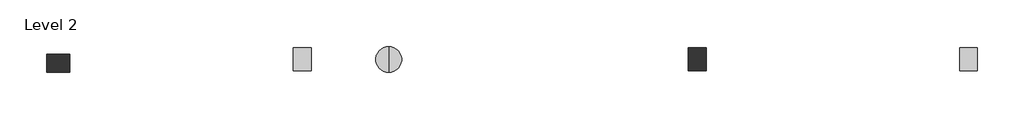
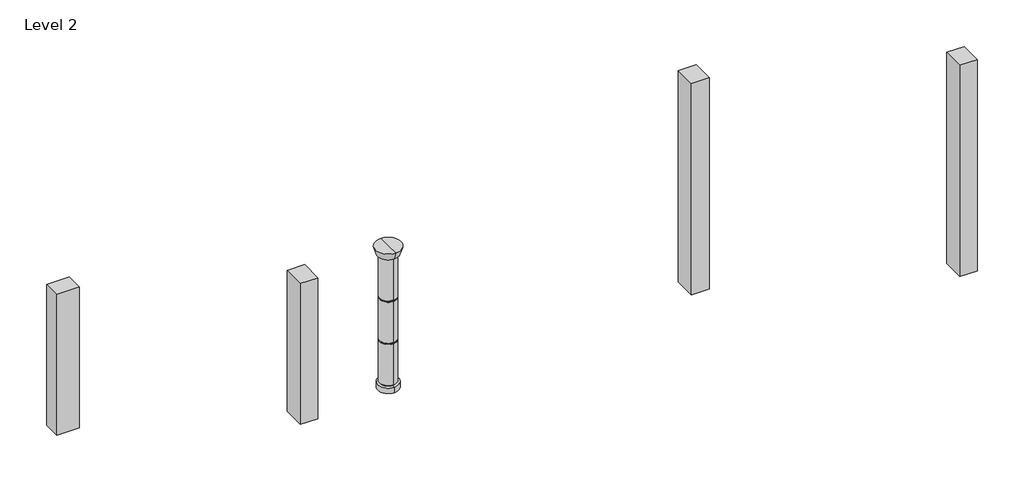
# One storey: 5 columns.
"""IFC4 building model written with IfcOpenShell, lengths in millimetres."""

import ifcopenshell
import ifcopenshell.guid

model = None  # the IFC model being written
_history = None  # IfcOwnerHistory: only IFC2X3 demands one
_inside = {}  # id of a spatial element -> (the spatial element, [elements in it])
_under = {}  # id of a project, library or spatial element -> (it, [spatial elements below it])
_declared = {}  # id of a project -> (the project, [libraries it declares])
_typed = {}  # id of a type object -> (the type object, [elements of that type])
_made_of = {}  # id of a material, layer set ... -> (it, [elements and type objects made of it])


def new_model(schema):
    """Start an empty IFC model of exactly this schema.

    Asked for "IFC4X3", IfcOpenShell would pick the latest addendum, in which some entities
    have other attributes; the version numbers below select the first issue.
    IFC2X3 requires an IfcOwnerHistory on every rooted entity: one is made here for all.
    """
    global model, _history
    if schema == "IFC4X3":
        model = ifcopenshell.file(schema_version=(4, 3, 0, 0))
    else:
        model = ifcopenshell.file(schema=schema)
    _inside.clear()
    _under.clear()
    _declared.clear()
    _typed.clear()
    _made_of.clear()
    _history = None
    if model.schema == "IFC2X3":
        org = make("IfcOrganization", Name="unknown")
        user = make(
            "IfcPersonAndOrganization",
            ThePerson=make("IfcPerson", FamilyName="unknown"),
            TheOrganization=org,
        )
        app = make(
            "IfcApplication",
            ApplicationDeveloper=org,
            Version="unknown",
            ApplicationFullName="unknown",
            ApplicationIdentifier="unknown",
        )
        _history = make(
            "IfcOwnerHistory",
            OwningUser=user,
            OwningApplication=app,
            ChangeAction="ADDED",
            CreationDate=0,
        )
    return model


def make(cls, **values):
    """One entity of the class cls with the attributes given. An attribute that is None is left unset."""
    return model.create_entity(
        cls, **{name: value for name, value in values.items() if value is not None}
    )


def rooted(cls, **values):
    """An entity with a GlobalId (a new one), such as an element, a storey or a relation."""
    return make(cls, GlobalId=ifcopenshell.guid.new(), OwnerHistory=_history, **values)


def si_unit(unit_type, name, prefix=None):
    """IfcSIUnit, for example si_unit("LENGTHUNIT", "METRE", prefix="MILLI")."""
    return make("IfcSIUnit", UnitType=unit_type, Prefix=prefix, Name=name)


def assignment(units):
    """IfcUnitAssignment: the units of a project."""
    return None if units is None else make("IfcUnitAssignment", Units=units)


def point(xyz):
    """IfcCartesianPoint."""
    return None if xyz is None else make("IfcCartesianPoint", Coordinates=xyz)


def direction(xyz):
    """IfcDirection."""
    return None if xyz is None else make("IfcDirection", DirectionRatios=xyz)


def frame(location, z_axis=None, x_axis=None):
    """IfcAxis2Placement3D, a coordinate frame: its origin and axes. An axis left out is left unset."""
    return make(
        "IfcAxis2Placement3D",
        Location=point(location),
        Axis=direction(z_axis),
        RefDirection=direction(x_axis),
    )


def origin():
    """The frame at (0, 0, 0) with its axes left unset."""
    return frame((0.0, 0.0, 0.0))


def origin_with_axes():
    """The frame at (0, 0, 0) with the z axis (0, 0, 1) and the x axis (1, 0, 0) written out."""
    return frame((0.0, 0.0, 0.0), z_axis=(0.0, 0.0, 1.0), x_axis=(1.0, 0.0, 0.0))


def place(relative_to, where):
    """IfcLocalPlacement: puts the frame where relative to a parent placement (None: the world)."""
    return make(
        "IfcLocalPlacement", PlacementRelTo=relative_to, RelativePlacement=where
    )


def context(
    kind, dimensions, precision=None, world=None, true_north=None, identifier=None
):
    """IfcGeometricRepresentationContext, for example the 3D "Model" context."""
    return make(
        "IfcGeometricRepresentationContext",
        ContextIdentifier=identifier,
        ContextType=kind,
        CoordinateSpaceDimension=dimensions,
        Precision=precision,
        WorldCoordinateSystem=world,
        TrueNorth=true_north,
    )


def project(units=None, contexts=None):
    """IfcProject with its units and contexts."""
    return rooted(
        "IfcProject",
        Name="project",
        RepresentationContexts=contexts,
        UnitsInContext=assignment(units),
    )


def spatial(cls, under=None, at=None, **own):
    """A site, building, storey or space (cls), placed at a placement, below another one or the project."""
    s = rooted(cls, ObjectPlacement=at, **own)
    if under is not None:
        _under.setdefault(under.id(), (under, []))[1].append(s)
    return s


def polyline(points):
    """IfcPolyline through the points."""
    return make("IfcPolyline", Points=[point(p) for p in points])


def circle_curve(where, radius):
    """IfcCircle in the frame where."""
    return make("IfcCircle", Position=where, Radius=radius)


def outline(outer, holes=None, kind="AREA"):
    """IfcArbitraryClosedProfileDef: a profile drawn as a closed curve; with holes, ...WithVoids."""
    if holes is None:
        return make("IfcArbitraryClosedProfileDef", ProfileType=kind, OuterCurve=outer)
    return make(
        "IfcArbitraryProfileDefWithVoids",
        ProfileType=kind,
        OuterCurve=outer,
        InnerCurves=holes,
    )


def extrude(swept, where, along, depth):
    """IfcExtrudedAreaSolid: the profile swept, set in the frame where, extruded along a direction by depth."""
    return make(
        "IfcExtrudedAreaSolid",
        SweptArea=swept,
        Position=where,
        ExtrudedDirection=direction(along),
        Depth=depth,
    )


def shape(context_of_items, identifier, shape_type, items):
    """IfcShapeRepresentation: the items that make up one representation, for example the "Body"."""
    return make(
        "IfcShapeRepresentation",
        ContextOfItems=context_of_items,
        RepresentationIdentifier=identifier,
        RepresentationType=shape_type,
        Items=items,
    )


def source(mapping_origin, context_of_items, identifier, shape_type, items):
    """IfcRepresentationMap: a shape defined once, which mapped items show again and again."""
    return make(
        "IfcRepresentationMap",
        MappingOrigin=mapping_origin,
        MappedRepresentation=shape(context_of_items, identifier, shape_type, items),
    )


def transform(
    local_origin,
    x_axis=None,
    y_axis=None,
    z_axis=None,
    scale=None,
    scale2=None,
    scale3=None,
    uniform=True,
):
    """IfcCartesianTransformationOperator3D, or its non-uniform kind. x_axis, y_axis, z_axis: its Axis1, 2, 3."""
    if uniform:
        return make(
            "IfcCartesianTransformationOperator3D",
            Axis1=direction(x_axis),
            Axis2=direction(y_axis),
            LocalOrigin=point(local_origin),
            Scale=scale,
            Axis3=direction(z_axis),
        )
    return make(
        "IfcCartesianTransformationOperator3DnonUniform",
        Axis1=direction(x_axis),
        Axis2=direction(y_axis),
        LocalOrigin=point(local_origin),
        Scale=scale,
        Axis3=direction(z_axis),
        Scale2=scale2,
        Scale3=scale3,
    )


def mapped(mapping_source, mapping_target):
    """IfcMappedItem: shows the shape of a source again, moved by a transform."""
    return make(
        "IfcMappedItem", MappingSource=mapping_source, MappingTarget=mapping_target
    )


def made_of(thing, what):
    """Note that an element or type object is made of a material, layer set ...; save() writes the relation."""
    if what is not None:
        _made_of.setdefault(what.id(), (what, []))[1].append(thing)
    return thing


def element(
    cls,
    number,
    at=None,
    inside=None,
    cuts=None,
    type_object=None,
    material=None,
    context=None,
    identifier="Body",
    shape_type=None,
    held_by="IfcProductDefinitionShape",
    body=None,
    shapes=None,
    **own,
):
    """One element of the class cls, such as IfcWall. Its Tag is "e" and its number.

    at: its placement. inside: the storey or other place that contains it. cuts: it is an
    opening in that element (IfcRelVoidsElement). A single representation is given by context,
    identifier, shape_type and body (its items); several are given by shapes. held_by: the class
    of the entity that holds the representations. save() writes the other relations.
    """
    e = rooted(cls, Tag="e%d" % number, ObjectPlacement=at, **own)
    if body is not None:
        shapes = [shape(context, identifier, shape_type, body)]
    if shapes is not None:
        e.Representation = make(held_by, Representations=shapes)
    if inside is not None:
        _inside.setdefault(inside.id(), (inside, []))[1].append(e)
    if cuts is not None:
        rooted(
            "IfcRelVoidsElement", RelatingBuildingElement=cuts, RelatedOpeningElement=e
        )
    if type_object is not None:
        _typed.setdefault(type_object.id(), (type_object, []))[1].append(e)
    return made_of(e, material)


def aggregate(whole, parts):
    """IfcRelAggregates: a whole, such as a stair, and the parts it consists of."""
    return rooted("IfcRelAggregates", RelatingObject=whole, RelatedObjects=parts)


def save(model, path):
    """Write the relations noted so far, then the file.

    IfcRelAggregates (storeys below a building ...), IfcRelContainedInSpatialStructure (elements
    in a storey), IfcRelDefinesByType, IfcRelAssociatesMaterial and IfcRelDeclares: one each for
    every whole, place, type object, material and project.
    """
    for whole, parts in _under.values():
        aggregate(whole, parts)
    for where, things in _inside.values():
        rooted(
            "IfcRelContainedInSpatialStructure",
            RelatedElements=things,
            RelatingStructure=where,
        )
    for kind, things in _typed.values():
        rooted("IfcRelDefinesByType", RelatedObjects=things, RelatingType=kind)
    for what, things in _made_of.values():
        rooted("IfcRelAssociatesMaterial", RelatedObjects=things, RelatingMaterial=what)
    for by, libraries in _declared.values():
        rooted("IfcRelDeclares", RelatingContext=by, RelatedDefinitions=libraries)
    model.write(path)


def plane_surface(at):
    """IfcPlane: the flat surface through the origin of the frame at, square to its z axis."""
    return make("IfcPlane", Position=at)


def cylinder_surface(at, radius):
    """IfcCylindricalSurface: all points at the distance radius from the z axis of the frame at."""
    return make("IfcCylindricalSurface", Position=at, Radius=radius)


def revolved_surface(curve, axis_point, axis_direction):
    """IfcSurfaceOfRevolution: the curve turned about the line through axis_point along axis_direction."""
    return make(
        "IfcSurfaceOfRevolution",
        SweptCurve=make("IfcArbitraryOpenProfileDef", ProfileType="CURVE", Curve=curve),
        AxisPosition=make("IfcAxis1Placement", Location=point(axis_point), Axis=direction(axis_direction)),
    )


def advanced_brep(points, edges, surfaces, faces):
    """IfcAdvancedBrep: a solid bounded by faces that lie on surfaces and meet in shared edges.

    An edge is (start, end): straight between two places in points (the first is 0);
    or (start, end, curve); or (start, end, curve, False) where it runs against its curve.
    A face is (place in surfaces, loops), or (place, loops, False) where it looks against
    its surface's normal. A loop lists edges by number (the first is 1), with a minus sign
    where the edge is run from its end to its start. The first loop is the outer one.
    """
    corners = [point(p) for p in points]
    vertices = [make("IfcVertexPoint", VertexGeometry=c) for c in corners]
    made = []
    for start, end, *more in edges:
        made.append(
            make(
                "IfcEdgeCurve",
                EdgeStart=vertices[start],
                EdgeEnd=vertices[end],
                EdgeGeometry=more[0] if more else make("IfcPolyline", Points=[corners[start], corners[end]]),
                SameSense=more[1] if len(more) > 1 else True,
            )
        )
    hull = []
    for where, loops, *sense in faces:
        bounds = []
        for j, loop in enumerate(loops):
            ring = [make("IfcOrientedEdge", EdgeElement=made[abs(k) - 1], Orientation=k > 0) for k in loop]
            bounds.append(
                make(
                    "IfcFaceOuterBound" if j == 0 else "IfcFaceBound",
                    Bound=make("IfcEdgeLoop", EdgeList=ring),
                    Orientation=True,
                )
            )
        hull.append(make("IfcAdvancedFace", Bounds=bounds, FaceSurface=surfaces[where], SameSense=sense[0] if sense else True))
    return make("IfcAdvancedBrep", Outer=make("IfcClosedShell", CfsFaces=hull))


def m_rectangular_column_475_x_610mm_712a9979(model_context):
    return source(origin(), model_context, "Body", "SweptSolid", [
        extrude(outline(polyline([(305.0, 237.5), (305.0, -237.5), (-305.0, -237.5), (-305.0, 237.5), (305.0, 237.5)])), origin_with_axes(), (0.0, 0.0, 1.0), 6000.0),
    ])


def m_rectangular_column_475_x_610mm_a7c237de(model_context):
    return source(origin(), model_context, "Body", "SweptSolid", [
        extrude(outline(polyline([(305.0, 237.5), (305.0, -237.5), (-305.0, -237.5), (-305.0, 237.5), (305.0, 237.5)])), frame((0.0, 0.0, -2000.0), z_axis=(0.0, 0.0, 1.0), x_axis=(1.0, 0.0, 0.0)), (0.0, 0.0, 1.0), 6000.0),
    ])


def m_rectangular_column_475_x_610mm_e62a7db6(model_context):
    return source(origin(), model_context, "Body", "SweptSolid", [
        extrude(outline(polyline([(305.0, 237.5), (305.0, -237.5), (-305.0, -237.5), (-305.0, 237.5), (305.0, 237.5)])), frame((0.0, 0.0, 2000.0), z_axis=(0.0, 0.0, 1.0), x_axis=(1.0, 0.0, 0.0)), (0.0, 0.0, 1.0), 4000.0),
    ])


def m_rectangular_column_475_x_610mm_b7c60445(model_context):
    return source(origin(), model_context, "Body", "SweptSolid", [
        extrude(outline(polyline([(305.0, 237.5), (305.0, -237.5), (-305.0, -237.5), (-305.0, 237.5), (305.0, 237.5)])), origin_with_axes(), (0.0, 0.0, 1.0), 4000.0),
    ])


def column_c029851a(model_context):
    return source(origin(), model_context, "Body", "AdvancedBrep", [
        advanced_brep(
        [(0.0, 0.0, 0.0), (-279.4, 0.0, 0.0), (279.4, 0.0, 0.0), (-279.4, 0.0, 152.4), (279.4, 0.0, 152.4), (203.2, 0.0, 1392.6), (-203.2, 0.0, 1392.6), (-228.6, 0.0, 1392.6), (228.6, 0.0, 1392.6), (-228.6, 0.0, 2556.6), (228.6, 0.0, 2556.6), (203.2, 0.0, 1354.5), (-203.2, 0.0, 1354.5), (228.6, 0.0, 1354.5), (-228.6, 0.0, 1354.5), (228.6, 0.0, 190.5), (-228.6, 0.0, 190.5), (203.2, 0.0, 190.5), (-203.2, 0.0, 190.5), (203.2, 0.0, 152.4), (-203.2, 0.0, 152.4), (279.4, 0.0, 3796.8), (-279.4, 0.0, 3796.8), (-342.9, 0.0, 4000.0), (342.9, 0.0, 4000.0), (0.0, 0.0, 4000.0), (203.2, 0.0, 3796.8), (-203.2, 0.0, 3796.8), (203.2, 0.0, 3758.7), (-203.2, 0.0, 3758.7), (228.6, 0.0, 3758.7), (-228.6, 0.0, 3758.7), (228.6, 0.0, 2594.7), (-228.6, 0.0, 2594.7), (203.2, 0.0, 2594.7), (-203.2, 0.0, 2594.7), (203.2, 0.0, 2556.6), (-203.2, 0.0, 2556.6)],
        [
            (0, 1),
            (1, 2, circle_curve(frame((0.0, 0.0, 0.0), z_axis=(0.0, 0.0, -1.0), x_axis=(-1.0, 0.0, 0.0)), 279.4)),
            (2, 0),
            (2, 1, circle_curve(frame((0.0, 0.0, 0.0), z_axis=(0.0, 0.0, -1.0), x_axis=(-1.0, 0.0, 0.0)), 279.4)),
            (1, 3),
            (3, 4, circle_curve(frame((0.0, 0.0, 152.4), z_axis=(0.0, 0.0, -1.0), x_axis=(-1.0, 0.0, 0.0)), 279.4)),
            (4, 2),
            (4, 3, circle_curve(frame((0.0, 0.0, 152.4), z_axis=(0.0, 0.0, -1.0), x_axis=(-1.0, 0.0, 0.0)), 279.4)),
            (5, 6, circle_curve(frame((0.0, 0.0, 1392.6), z_axis=(0.0, 0.0, 1.0), x_axis=(-1.0, 0.0, 0.0)), 203.2)),
            (6, 7),
            (7, 8, circle_curve(frame((0.0, 0.0, 1392.6), z_axis=(0.0, 0.0, -1.0), x_axis=(-1.0, 0.0, 0.0)), 228.6)),
            (8, 5),
            (7, 9),
            (9, 10, circle_curve(frame((0.0, 0.0, 2556.6), z_axis=(0.0, 0.0, -1.0), x_axis=(-1.0, 0.0, 0.0)), 228.6)),
            (10, 8),
            (7, 8, circle_curve(frame((0.0, 0.0, 1392.6), z_axis=(0.0, 0.0, 1.0), x_axis=(-1.0, 0.0, 0.0)), 228.6)),
            (10, 9, circle_curve(frame((0.0, 0.0, 2556.6), z_axis=(0.0, 0.0, -1.0), x_axis=(-1.0, 0.0, 0.0)), 228.6)),
            (6, 5, circle_curve(frame((0.0, 0.0, 1392.6), z_axis=(0.0, 0.0, 1.0), x_axis=(-1.0, 0.0, 0.0)), 203.2)),
            (11, 12, circle_curve(frame((0.0, 0.0, 1354.5), z_axis=(0.0, 0.0, 1.0), x_axis=(-1.0, 0.0, 0.0)), 203.2)),
            (12, 6),
            (5, 11),
            (12, 11, circle_curve(frame((0.0, 0.0, 1354.5), z_axis=(0.0, 0.0, 1.0), x_axis=(-1.0, 0.0, 0.0)), 203.2)),
            (13, 14, circle_curve(frame((0.0, 0.0, 1354.5), z_axis=(0.0, 0.0, 1.0), x_axis=(-1.0, 0.0, 0.0)), 228.6)),
            (14, 12),
            (11, 13),
            (14, 13, circle_curve(frame((0.0, 0.0, 1354.5), z_axis=(0.0, 0.0, 1.0), x_axis=(-1.0, 0.0, 0.0)), 228.6)),
            (15, 16, circle_curve(frame((0.0, 0.0, 190.5), z_axis=(0.0, 0.0, 1.0), x_axis=(-1.0, 0.0, 0.0)), 228.6)),
            (16, 14),
            (13, 15),
            (16, 15, circle_curve(frame((0.0, 0.0, 190.5), z_axis=(0.0, 0.0, 1.0), x_axis=(-1.0, 0.0, 0.0)), 228.6)),
            (17, 18, circle_curve(frame((0.0, 0.0, 190.5), z_axis=(0.0, 0.0, 1.0), x_axis=(-1.0, 0.0, 0.0)), 203.2)),
            (18, 16),
            (15, 17),
            (18, 17, circle_curve(frame((0.0, 0.0, 190.5), z_axis=(0.0, 0.0, 1.0), x_axis=(-1.0, 0.0, 0.0)), 203.2)),
            (19, 20, circle_curve(frame((0.0, 0.0, 152.4), z_axis=(0.0, 0.0, 1.0), x_axis=(-1.0, 0.0, 0.0)), 203.2)),
            (20, 18),
            (17, 19),
            (20, 19, circle_curve(frame((0.0, 0.0, 152.4), z_axis=(0.0, 0.0, 1.0), x_axis=(-1.0, 0.0, 0.0)), 203.2)),
            (3, 20),
            (19, 4),
            (21, 22, circle_curve(frame((0.0, 0.0, 3796.8), z_axis=(0.0, 0.0, 1.0), x_axis=(-1.0, 0.0, 0.0)), 279.4)),
            (22, 23),
            (23, 24, circle_curve(frame((0.0, 0.0, 4000.0), z_axis=(0.0, 0.0, -1.0), x_axis=(-1.0, 0.0, 0.0)), 342.9)),
            (24, 21),
            (23, 25),
            (25, 24),
            (23, 24, circle_curve(frame((0.0, 0.0, 4000.0), z_axis=(0.0, 0.0, 1.0), x_axis=(-1.0, 0.0, 0.0)), 342.9)),
            (22, 21, circle_curve(frame((0.0, 0.0, 3796.8), z_axis=(0.0, 0.0, 1.0), x_axis=(-1.0, 0.0, 0.0)), 279.4)),
            (26, 27, circle_curve(frame((0.0, 0.0, 3796.8), z_axis=(0.0, 0.0, 1.0), x_axis=(-1.0, 0.0, 0.0)), 203.2)),
            (27, 22),
            (21, 26),
            (27, 26, circle_curve(frame((0.0, 0.0, 3796.8), z_axis=(0.0, 0.0, 1.0), x_axis=(-1.0, 0.0, 0.0)), 203.2)),
            (28, 29, circle_curve(frame((0.0, 0.0, 3758.7), z_axis=(0.0, 0.0, 1.0), x_axis=(-1.0, 0.0, 0.0)), 203.2)),
            (29, 27),
            (26, 28),
            (29, 28, circle_curve(frame((0.0, 0.0, 3758.7), z_axis=(0.0, 0.0, 1.0), x_axis=(-1.0, 0.0, 0.0)), 203.2)),
            (30, 31, circle_curve(frame((0.0, 0.0, 3758.7), z_axis=(0.0, 0.0, 1.0), x_axis=(-1.0, 0.0, 0.0)), 228.6)),
            (31, 29),
            (28, 30),
            (31, 30, circle_curve(frame((0.0, 0.0, 3758.7), z_axis=(0.0, 0.0, 1.0), x_axis=(-1.0, 0.0, 0.0)), 228.6)),
            (32, 33, circle_curve(frame((0.0, 0.0, 2594.7), z_axis=(0.0, 0.0, 1.0), x_axis=(-1.0, 0.0, 0.0)), 228.6)),
            (33, 31),
            (30, 32),
            (33, 32, circle_curve(frame((0.0, 0.0, 2594.7), z_axis=(0.0, 0.0, 1.0), x_axis=(-1.0, 0.0, 0.0)), 228.6)),
            (34, 35, circle_curve(frame((0.0, 0.0, 2594.7), z_axis=(0.0, 0.0, 1.0), x_axis=(-1.0, 0.0, 0.0)), 203.2)),
            (35, 33),
            (32, 34),
            (35, 34, circle_curve(frame((0.0, 0.0, 2594.7), z_axis=(0.0, 0.0, 1.0), x_axis=(-1.0, 0.0, 0.0)), 203.2)),
            (36, 37, circle_curve(frame((0.0, 0.0, 2556.6), z_axis=(0.0, 0.0, 1.0), x_axis=(-1.0, 0.0, 0.0)), 203.2)),
            (37, 35),
            (34, 36),
            (37, 36, circle_curve(frame((0.0, 0.0, 2556.6), z_axis=(0.0, 0.0, 1.0), x_axis=(-1.0, 0.0, 0.0)), 203.2)),
            (9, 37),
            (36, 10),
        ],
        [
            plane_surface(frame((0.0, 0.0, 0.0), z_axis=(0.0, 0.0, -1.0), x_axis=(-1.0, 0.0, 0.0))),
            cylinder_surface(frame((0.0, 0.0, 4000.0), z_axis=(0.0, 0.0, -1.0), x_axis=(-1.0, 0.0, 0.0)), 279.4),
            plane_surface(frame((0.0, 0.0, 1392.6), z_axis=(0.0, 0.0, -1.0), x_axis=(-1.0, 0.0, 0.0))),
            cylinder_surface(frame((0.0, 0.0, 4000.0), z_axis=(0.0, 0.0, -1.0), x_axis=(-1.0, 0.0, 0.0)), 228.6),
            cylinder_surface(frame((0.0, 0.0, 4000.0), z_axis=(0.0, 0.0, -1.0), x_axis=(-1.0, 0.0, 0.0)), 203.2),
            plane_surface(frame((0.0, 0.0, 1354.5), z_axis=(0.0, 0.0, 1.0), x_axis=(-1.0, 0.0, 0.0))),
            plane_surface(frame((0.0, 0.0, 190.5), z_axis=(0.0, 0.0, -1.0), x_axis=(-1.0, 0.0, 0.0))),
            plane_surface(frame((0.0, 0.0, 152.4), z_axis=(0.0, 0.0, 1.0), x_axis=(-1.0, 0.0, 0.0))),
            revolved_surface(polyline([(-342.9, 0.0, 4000.0), (-279.4, 0.0, 3796.8)]), (0.0, 0.0, 4000.0), (0.0, 0.0, -1.0)),
            plane_surface(frame((0.0, 0.0, 4000.0), z_axis=(0.0, 0.0, 1.0), x_axis=(-1.0, 0.0, 0.0))),
            plane_surface(frame((0.0, 0.0, 3796.8), z_axis=(0.0, 0.0, -1.0), x_axis=(-1.0, 0.0, 0.0))),
            plane_surface(frame((0.0, 0.0, 3758.7), z_axis=(0.0, 0.0, 1.0), x_axis=(-1.0, 0.0, 0.0))),
            plane_surface(frame((0.0, 0.0, 2594.7), z_axis=(0.0, 0.0, -1.0), x_axis=(-1.0, 0.0, 0.0))),
            plane_surface(frame((0.0, 0.0, 2556.6), z_axis=(0.0, 0.0, 1.0), x_axis=(-1.0, 0.0, 0.0))),
        ],
        [
            (0, [[1, 2, 3]]),
            (0, [[-3, 4, -1]]),
            (1, [[-2, 5, 6, 7]]),
            (1, [[-4, -7, 8, -5]]),
            (2, [[9, 10, 11, 12]]),
            (3, [[-11, 13, 14, 15]]),
            (3, [[16, -15, 17, -13]]),
            (2, [[18, -12, -16, -10]]),
            (4, [[19, 20, -9, 21]]),
            (4, [[22, -21, -18, -20]]),
            (5, [[23, 24, -19, 25]]),
            (5, [[26, -25, -22, -24]]),
            (3, [[27, 28, -23, 29]]),
            (3, [[30, -29, -26, -28]]),
            (6, [[31, 32, -27, 33]]),
            (6, [[34, -33, -30, -32]]),
            (4, [[35, 36, -31, 37]]),
            (4, [[38, -37, -34, -36]]),
            (7, [[-6, 39, -35, 40]]),
            (7, [[-8, -40, -38, -39]]),
            (8, [[41, 42, 43, 44]]),
            (9, [[-43, 45, 46]]),
            (9, [[47, -46, -45]]),
            (8, [[48, -44, -47, -42]]),
            (10, [[49, 50, -41, 51]]),
            (10, [[52, -51, -48, -50]]),
            (4, [[53, 54, -49, 55]]),
            (4, [[56, -55, -52, -54]]),
            (11, [[57, 58, -53, 59]]),
            (11, [[60, -59, -56, -58]]),
            (3, [[61, 62, -57, 63]]),
            (3, [[64, -63, -60, -62]]),
            (12, [[65, 66, -61, 67]]),
            (12, [[68, -67, -64, -66]]),
            (4, [[69, 70, -65, 71]]),
            (4, [[72, -71, -68, -70]]),
            (13, [[-14, 73, -69, 74]]),
            (13, [[-17, -74, -72, -73]]),
        ],
    ),
    ])


model = new_model("IFC4")

# Units and contexts
model_context = context("Model", 3, world=origin())
ifc_project = project(units=[si_unit("LENGTHUNIT", "METRE", prefix="MILLI")], contexts=[model_context])

# Site, building, storey
site = spatial("IfcSite", under=ifc_project)
building = spatial("IfcBuilding", under=site)
storey = spatial("IfcBuildingStorey", under=building, Name="Level 2", Elevation=4000.0)

# Columns
placement = place(None, origin())
m_rectangular_column_475_x_610mm_shape = m_rectangular_column_475_x_610mm_712a9979(model_context)
element("IfcColumn", 1, ObjectType="M_Rectangular Column : 475 x 610mm", at=placement, inside=storey, context=model_context, shape_type="MappedRepresentation", body=[
    mapped(m_rectangular_column_475_x_610mm_shape, transform((-672.9984463, 10294.8525449, 0.0), x_axis=(0.0, 1.0, 0.0), y_axis=(-1.0, 0.0, 0.0), z_axis=(0.0, 0.0, 1.0))),
])
m_rectangular_column_475_x_610mm_2_shape = m_rectangular_column_475_x_610mm_a7c237de(model_context)
element("IfcColumn", 2, ObjectType="M_Rectangular Column : 475 x 610mm", at=placement, inside=storey, context=model_context, shape_type="MappedRepresentation", body=[
    mapped(m_rectangular_column_475_x_610mm_2_shape, transform((6527.0015537, 10294.8525449, 0.0), x_axis=(0.0, 1.0, 0.0), y_axis=(-1.0, 0.0, 0.0), z_axis=(0.0, 0.0, 1.0))),
])
m_rectangular_column_475_x_610mm_3_shape = m_rectangular_column_475_x_610mm_e62a7db6(model_context)
element("IfcColumn", 3, ObjectType="M_Rectangular Column : 475 x 610mm", at=placement, inside=storey, context=model_context, shape_type="MappedRepresentation", body=[
    mapped(m_rectangular_column_475_x_610mm_3_shape, transform((-17655.4655243, 10194.8525449, 0.0), x_axis=(1.0, 0.0, 0.0), y_axis=(0.0, 1.0, 0.0), z_axis=(0.0, 0.0, 1.0))),
])
m_rectangular_column_475_x_610mm_4_shape = m_rectangular_column_475_x_610mm_b7c60445(model_context)
element("IfcColumn", 4, ObjectType="M_Rectangular Column : 475 x 610mm", at=placement, inside=storey, context=model_context, shape_type="MappedRepresentation", body=[
    mapped(m_rectangular_column_475_x_610mm_4_shape, transform((-11172.9984463, 10294.8525449, 0.0), x_axis=(0.0, 1.0, 0.0), y_axis=(-1.0, 0.0, 0.0), z_axis=(0.0, 0.0, 1.0))),
])
column_shape = column_c029851a(model_context)
element("IfcColumn", 5, ObjectType="Metal Clad Column : 18\"", at=placement, inside=storey, context=model_context, shape_type="MappedRepresentation", body=[
    mapped(column_shape, transform((-8872.9984463, 10294.8525449, 0.0), x_axis=(0.0, 1.0, 0.0), y_axis=(-1.0, 0.0, 0.0), z_axis=(0.0, 0.0, 1.0))),
])

save(model, "model.ifc")

# Revit data of these elements
# Type "M_Rectangular Column : 475 x 610mm"
#   Depth = 475 mm
#   Offset Base = 0 mm
#   Offset Top = 0 mm
#   Width = 610 mm
#   Material = Copper
# Type "Metal Clad Column : 18\""
#   Assembly Code = "B1010200"
#   Base = 152.4 mm
#   Capital = 203.2 mm
#   Diameter = 457.2 mm
#   Joint Depth = 25.4 mm
#   Joint Width = 38.1 mm
#   Offset base level = 0 mm
#   Offset top level = 0 mm
#   Material = Aluminum
# Element 1 (IfcColumn, "M_Rectangular Column : 475 x 610mm")
#   SpeckleObjectUpdateDescription = "No changes yet"
#   SpeckleObjectTestNumber = 8
#   Phase Created = New Construction
#   Materials on its faces: "Copper"
# Element 2 (IfcColumn, "M_Rectangular Column : 475 x 610mm")
#   SpeckleObjectUpdateDescription = "No changes yet"
#   SpeckleObjectTestNumber = 10
#   Phase Created = New Construction
#   Materials on its faces: "Copper"
# Element 3 (IfcColumn, "M_Rectangular Column : 475 x 610mm")
#   SpeckleObjectUpdateDescription = "reference different levels"
#   SpeckleObjectTestNumber = 1
#   Phase Created = New Construction
#   Materials on its faces: "Copper"
# Element 4 (IfcColumn, "M_Rectangular Column : 475 x 610mm")
#   SpeckleObjectUpdateDescription = "flip column ends"
#   SpeckleObjectTestNumber = 4
#   Phase Created = New Construction
#   Materials on its faces: "Copper"
# Element 5 (IfcColumn, "Metal Clad Column : 18\"")
#   SpeckleObjectUpdateDescription = "change column type"
#   SpeckleObjectTestNumber = 5
#   Phase Created = New Construction
#   Materials on its faces: "Aluminum"
# Materials
#   "Copper": class "Metal", colour RGB 0 0 0, transparency 0, Description = "Copper, matte finish", Cost = 0
#   "Aluminum": class "Metal", colour RGB 247 247 247, transparency 0, Description = "Aluminum 6061", Cost = 0
